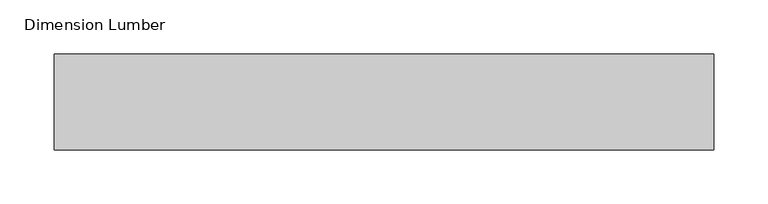
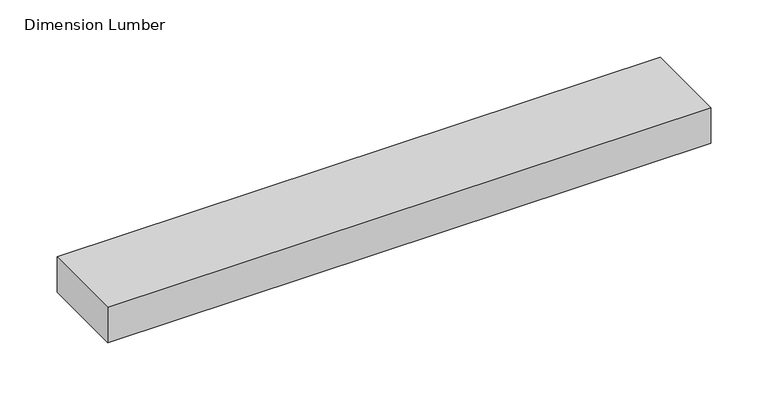
"""IFC4 building model written with IfcOpenShell, lengths in millimetres: beam geometry, Dimension Lumber : Opening Plate 2*4 Exterior."""

from ifc_helpers import new_model, si_unit, frame, origin, place, context, project, spatial, polyline, outline, extrude, source, transform, mapped, element, save


def dimension_lumber_b6f9b94d(model_context):
    return source(origin(), model_context, "Body", "SweptSolid", [
        extrude(outline(polyline([(295.275, 44.45), (295.275, -44.45), (-314.3249994, -44.45), (-314.3249994, 44.45), (295.275, 44.45)])), frame((0.0, 0.0, -19.05), z_axis=(0.0, 0.0, 1.0), x_axis=(1.0, 0.0, 0.0)), (0.0, 0.0, 1.0), 38.1),
    ])


if __name__ == "__main__":
    model = new_model("IFC4")
    model_context = context("Model", 3, world=origin())
    ifc_project = project(units=[si_unit("LENGTHUNIT", "METRE", prefix="MILLI")], contexts=[model_context])
    site = spatial("IfcSite", under=ifc_project)
    building = spatial("IfcBuilding", under=site)
    placement = place(None, origin())
    dimension_lumber_shape = dimension_lumber_b6f9b94d(model_context)
    element("IfcBeam", 1, ObjectType="Dimension Lumber : Opening Plate 2*4 Exterior", at=placement, inside=building, context=model_context, shape_type="MappedRepresentation", body=[
        mapped(dimension_lumber_shape, transform((0.0, 0.0, 0.0), x_axis=(1.0, 0.0, 0.0), y_axis=(0.0, 1.0, 0.0), z_axis=(0.0, 0.0, 1.0))),
    ])
    save(model, "model.ifc")

# Revit data of these elements
# Type "Dimension Lumber : Opening Plate 2*4 Exterior"
#   Assembly Code = "B10"
#   A = 0.0364583 SF
#   Length [instance default] = 5' - 0"
#   b = 0' - 3 1/2"
#   d = 0' - 1 1/2"
#   Structural Material [instance default] = Softwood, Lumber
# Element 1 (IfcBeam, "Dimension Lumber : Opening Plate 2*4 Exterior")
#   Structural Material = Douglas Fir #2
#   Materials on its faces: "Douglas Fir #2"
# Materials
#   "Softwood, Lumber": class "Wood", colour RGB 223 192 134, transparency 0, Description = "Pinus Echinata", Cost = 0
#   "Douglas Fir #2": class "Wood", colour RGB 223 192 134, transparency 0, Description = "Pinus Echinata", Cost = 0
